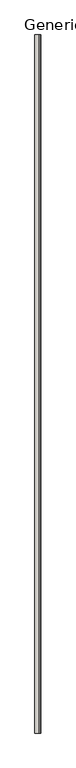
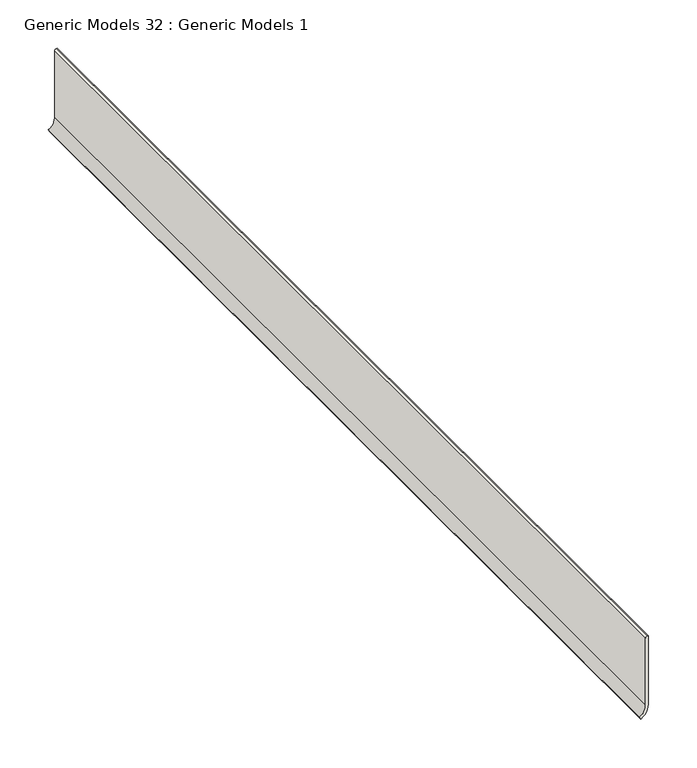
"""IFC4 building model written with IfcOpenShell, lengths in millimetres: wall geometry, Generic Models 32 : Generic Models 1."""

from ifc_helpers import new_model, si_unit, point, frame, frame_2d, origin, place, context, project, spatial, polyline, circle_curve, trimmed, segment, composite_curve, outline, extrude, source, transform, mapped, element, save


def generic_models_32_generic_models_1_c5b7b2a8(model_context):
    return source(origin(), model_context, "Body", "SweptSolid", [
        extrude(outline(composite_curve([segment(polyline([(101.6, 49676.05), (101.6, 49674.9618018)]), True, "CONTINUOUS"), segment(trimmed(circle_curve(frame_2d((99.5131982, 49674.9618018)), 2.0868018), [point((101.6, 49674.9618018))], [point((99.5131982, 49672.875))], False, "CARTESIAN"), True, "CONTINUOUS"), segment(polyline([(99.5131982, 49672.875), (15.4496307, 49672.875)]), True, "CONTINUOUS"), segment(trimmed(circle_curve(frame_2d((15.4496307, 49658.2103032)), 14.6646968), [point((15.4496307, 49672.875))], [point((2.7496307, 49665.5426516))], True, "CARTESIAN"), True, "CONTINUOUS"), segment(polyline([(2.7496307, 49665.5426516), (0.0, 49667.1301516)]), True, "CONTINUOUS"), segment(trimmed(circle_curve(frame_2d((15.4496307, 49658.2103032)), 17.8396968), [point((0.0, 49667.1301516))], [point((15.4496307, 49676.05))], False, "CARTESIAN"), True, "CONTINUOUS"), segment(polyline([(15.4496307, 49676.05), (101.6, 49676.05)]), True, "CONTINUOUS")], self_intersect=False)), frame((0.0, 0.0, 0.0), z_axis=(0.0, 1.0, 0.0), x_axis=(0.0, 0.0, 1.0)), (0.0, 0.0, 1.0), 1219.2),
    ])


if __name__ == "__main__":
    model = new_model("IFC4")
    model_context = context("Model", 3, world=origin())
    ifc_project = project(units=[si_unit("LENGTHUNIT", "METRE", prefix="MILLI")], contexts=[model_context])
    site = spatial("IfcSite", under=ifc_project)
    building = spatial("IfcBuilding", under=site)
    placement = place(None, origin())
    generic_models_32_generic_models_1_shape = generic_models_32_generic_models_1_c5b7b2a8(model_context)
    element("IfcWall", 1, ObjectType="Generic Models 32 : Generic Models 1", at=placement, inside=building, context=model_context, shape_type="MappedRepresentation", body=[
        mapped(generic_models_32_generic_models_1_shape, transform((0.0, 0.0, 0.0), x_axis=(1.0, 0.0, 0.0), y_axis=(0.0, 1.0, 0.0), z_axis=(0.0, 0.0, 1.0))),
    ])
    save(model, "model.ifc")

# Revit data of these elements
# Element 1 (IfcWall, "Generic Models 32 : Generic Models 1")
#   Materials on its faces: "WALL BASE AS SCHEDULED"
# Materials
#   "WALL BASE AS SCHEDULED": class "Generic", colour RGB 120 120 120, transparency 0, Cost = 0
